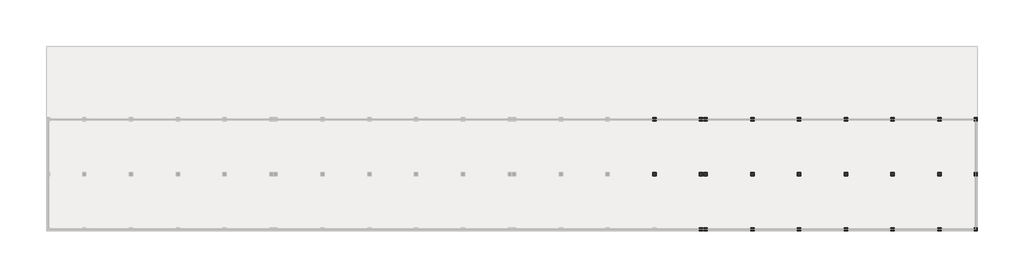
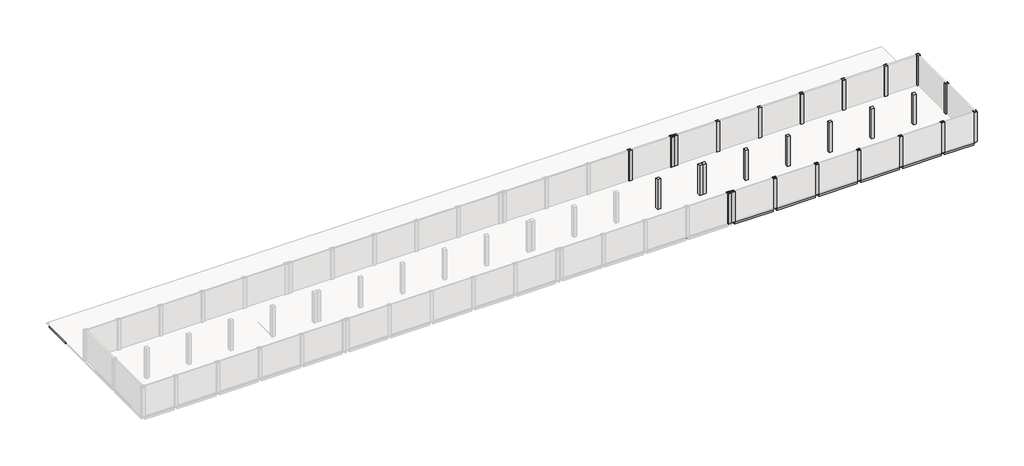
# One storey, part 3 of 4: 52 beams, 26 columns.
"""IFC4 building model written with IfcOpenShell, lengths in millimetres."""

import ifcopenshell
import ifcopenshell.guid

model = None  # the IFC model being written
_history = None  # IfcOwnerHistory: only IFC2X3 demands one
_inside = {}  # id of a spatial element -> (the spatial element, [elements in it])
_under = {}  # id of a project, library or spatial element -> (it, [spatial elements below it])
_declared = {}  # id of a project -> (the project, [libraries it declares])
_typed = {}  # id of a type object -> (the type object, [elements of that type])
_made_of = {}  # id of a material, layer set ... -> (it, [elements and type objects made of it])


def new_model(schema):
    """Start an empty IFC model of exactly this schema.

    Asked for "IFC4X3", IfcOpenShell would pick the latest addendum, in which some entities
    have other attributes; the version numbers below select the first issue.
    IFC2X3 requires an IfcOwnerHistory on every rooted entity: one is made here for all.
    """
    global model, _history
    if schema == "IFC4X3":
        model = ifcopenshell.file(schema_version=(4, 3, 0, 0))
    else:
        model = ifcopenshell.file(schema=schema)
    _inside.clear()
    _under.clear()
    _declared.clear()
    _typed.clear()
    _made_of.clear()
    _history = None
    if model.schema == "IFC2X3":
        org = make("IfcOrganization", Name="unknown")
        user = make(
            "IfcPersonAndOrganization",
            ThePerson=make("IfcPerson", FamilyName="unknown"),
            TheOrganization=org,
        )
        app = make(
            "IfcApplication",
            ApplicationDeveloper=org,
            Version="unknown",
            ApplicationFullName="unknown",
            ApplicationIdentifier="unknown",
        )
        _history = make(
            "IfcOwnerHistory",
            OwningUser=user,
            OwningApplication=app,
            ChangeAction="ADDED",
            CreationDate=0,
        )
    return model


def make(cls, **values):
    """One entity of the class cls with the attributes given. An attribute that is None is left unset."""
    return model.create_entity(
        cls, **{name: value for name, value in values.items() if value is not None}
    )


def rooted(cls, **values):
    """An entity with a GlobalId (a new one), such as an element, a storey or a relation."""
    return make(cls, GlobalId=ifcopenshell.guid.new(), OwnerHistory=_history, **values)


def si_unit(unit_type, name, prefix=None):
    """IfcSIUnit, for example si_unit("LENGTHUNIT", "METRE", prefix="MILLI")."""
    return make("IfcSIUnit", UnitType=unit_type, Prefix=prefix, Name=name)


def assignment(units):
    """IfcUnitAssignment: the units of a project."""
    return None if units is None else make("IfcUnitAssignment", Units=units)


def point(xyz):
    """IfcCartesianPoint."""
    return None if xyz is None else make("IfcCartesianPoint", Coordinates=xyz)


def direction(xyz):
    """IfcDirection."""
    return None if xyz is None else make("IfcDirection", DirectionRatios=xyz)


def frame(location, z_axis=None, x_axis=None):
    """IfcAxis2Placement3D, a coordinate frame: its origin and axes. An axis left out is left unset."""
    return make(
        "IfcAxis2Placement3D",
        Location=point(location),
        Axis=direction(z_axis),
        RefDirection=direction(x_axis),
    )


def origin():
    """The frame at (0, 0, 0) with its axes left unset."""
    return frame((0.0, 0.0, 0.0))


def place(relative_to, where):
    """IfcLocalPlacement: puts the frame where relative to a parent placement (None: the world)."""
    return make(
        "IfcLocalPlacement", PlacementRelTo=relative_to, RelativePlacement=where
    )


def context(
    kind, dimensions, precision=None, world=None, true_north=None, identifier=None
):
    """IfcGeometricRepresentationContext, for example the 3D "Model" context."""
    return make(
        "IfcGeometricRepresentationContext",
        ContextIdentifier=identifier,
        ContextType=kind,
        CoordinateSpaceDimension=dimensions,
        Precision=precision,
        WorldCoordinateSystem=world,
        TrueNorth=true_north,
    )


def project(units=None, contexts=None):
    """IfcProject with its units and contexts."""
    return rooted(
        "IfcProject",
        Name="project",
        RepresentationContexts=contexts,
        UnitsInContext=assignment(units),
    )


def spatial(cls, under=None, at=None, **own):
    """A site, building, storey or space (cls), placed at a placement, below another one or the project."""
    s = rooted(cls, ObjectPlacement=at, **own)
    if under is not None:
        _under.setdefault(under.id(), (under, []))[1].append(s)
    return s


def polyline(points):
    """IfcPolyline through the points."""
    return make("IfcPolyline", Points=[point(p) for p in points])


def outline(outer, holes=None, kind="AREA"):
    """IfcArbitraryClosedProfileDef: a profile drawn as a closed curve; with holes, ...WithVoids."""
    if holes is None:
        return make("IfcArbitraryClosedProfileDef", ProfileType=kind, OuterCurve=outer)
    return make(
        "IfcArbitraryProfileDefWithVoids",
        ProfileType=kind,
        OuterCurve=outer,
        InnerCurves=holes,
    )


def extrude(swept, where, along, depth):
    """IfcExtrudedAreaSolid: the profile swept, set in the frame where, extruded along a direction by depth."""
    return make(
        "IfcExtrudedAreaSolid",
        SweptArea=swept,
        Position=where,
        ExtrudedDirection=direction(along),
        Depth=depth,
    )


def shape(context_of_items, identifier, shape_type, items):
    """IfcShapeRepresentation: the items that make up one representation, for example the "Body"."""
    return make(
        "IfcShapeRepresentation",
        ContextOfItems=context_of_items,
        RepresentationIdentifier=identifier,
        RepresentationType=shape_type,
        Items=items,
    )


def made_of(thing, what):
    """Note that an element or type object is made of a material, layer set ...; save() writes the relation."""
    if what is not None:
        _made_of.setdefault(what.id(), (what, []))[1].append(thing)
    return thing


def element(
    cls,
    number,
    at=None,
    inside=None,
    cuts=None,
    type_object=None,
    material=None,
    context=None,
    identifier="Body",
    shape_type=None,
    held_by="IfcProductDefinitionShape",
    body=None,
    shapes=None,
    **own,
):
    """One element of the class cls, such as IfcWall. Its Tag is "e" and its number.

    at: its placement. inside: the storey or other place that contains it. cuts: it is an
    opening in that element (IfcRelVoidsElement). A single representation is given by context,
    identifier, shape_type and body (its items); several are given by shapes. held_by: the class
    of the entity that holds the representations. save() writes the other relations.
    """
    e = rooted(cls, Tag="e%d" % number, ObjectPlacement=at, **own)
    if body is not None:
        shapes = [shape(context, identifier, shape_type, body)]
    if shapes is not None:
        e.Representation = make(held_by, Representations=shapes)
    if inside is not None:
        _inside.setdefault(inside.id(), (inside, []))[1].append(e)
    if cuts is not None:
        rooted(
            "IfcRelVoidsElement", RelatingBuildingElement=cuts, RelatedOpeningElement=e
        )
    if type_object is not None:
        _typed.setdefault(type_object.id(), (type_object, []))[1].append(e)
    return made_of(e, material)


def aggregate(whole, parts):
    """IfcRelAggregates: a whole, such as a stair, and the parts it consists of."""
    return rooted("IfcRelAggregates", RelatingObject=whole, RelatedObjects=parts)


def save(model, path):
    """Write the relations noted so far, then the file.

    IfcRelAggregates (storeys below a building ...), IfcRelContainedInSpatialStructure (elements
    in a storey), IfcRelDefinesByType, IfcRelAssociatesMaterial and IfcRelDeclares: one each for
    every whole, place, type object, material and project.
    """
    for whole, parts in _under.values():
        aggregate(whole, parts)
    for where, things in _inside.values():
        rooted(
            "IfcRelContainedInSpatialStructure",
            RelatedElements=things,
            RelatingStructure=where,
        )
    for kind, things in _typed.values():
        rooted("IfcRelDefinesByType", RelatedObjects=things, RelatingType=kind)
    for what, things in _made_of.values():
        rooted("IfcRelAssociatesMaterial", RelatedObjects=things, RelatingMaterial=what)
    for by, libraries in _declared.values():
        rooted("IfcRelDeclares", RelatingContext=by, RelatedDefinitions=libraries)
    model.write(path)


model = new_model("IFC4")

# Units and contexts
model_context = context("Model", 3, world=origin())
ifc_project = project(units=[si_unit("LENGTHUNIT", "METRE", prefix="MILLI")], contexts=[model_context])

# Site, building, storey
site = spatial("IfcSite", under=ifc_project)
building = spatial("IfcBuilding", under=site)
storey = spatial("IfcBuildingStorey", under=building, Name="03_T.O.C_1", Elevation=6949.9618634)

# Beams
placement = place(None, origin())
element("IfcBeam", 1, ObjectType="RC Beam_Rectangular : H_SB_AR_S16_B300xH600", at=placement, inside=storey, context=model_context, shape_type="SweptSolid", body=[
    extrude(outline(polyline([(93930.0, -6150.4791411), (93930.0, -5850.4791411), (101530.0, -5850.4791411), (101530.0, -6150.4791411), (93930.0, -6150.4791411)])), frame((0.0, 0.0, 6349.9618634), z_axis=(0.0, 0.0, 1.0), x_axis=(1.0, 0.0, 0.0)), (0.0, 0.0, 1.0), 499.0),
])
element("IfcBeam", 2, ObjectType="RC Beam_Rectangular : H_SB_AR_S16_B300xH600", at=placement, inside=storey, context=model_context, shape_type="SweptSolid", body=[
    extrude(outline(polyline([(102130.0, -6150.4791411), (102130.0, -5850.4791411), (109730.0, -5850.4791411), (109730.0, -6150.4791411), (102130.0, -6150.4791411)])), frame((0.0, 0.0, 6349.9618634), z_axis=(0.0, 0.0, 1.0), x_axis=(1.0, 0.0, 0.0)), (0.0, 0.0, 1.0), 499.0),
])
element("IfcBeam", 3, ObjectType="RC Beam_Rectangular : H_SB_AR_S16_B300xH600", at=placement, inside=storey, context=model_context, shape_type="SweptSolid", body=[
    extrude(outline(polyline([(110330.0, -6150.4791411), (110330.0, -5850.4791411), (110480.0, -5850.4791411), (110480.0, -6150.4791411), (110330.0, -6150.4791411)])), frame((0.0, 0.0, 6349.9618634), z_axis=(0.0, 0.0, 1.0), x_axis=(1.0, 0.0, 0.0)), (0.0, 0.0, 1.0), 499.0),
])
element("IfcBeam", 4, ObjectType="RC Beam_Rectangular : H_SB_AR_S16_B300xH600", at=placement, inside=storey, context=model_context, shape_type="SweptSolid", body=[
    extrude(outline(polyline([(111080.0, -6150.4791411), (111080.0, -5850.4791411), (118680.0, -5850.4791411), (118680.0, -6150.4791411), (111080.0, -6150.4791411)])), frame((0.0, 0.0, 6349.9618634), z_axis=(0.0, 0.0, 1.0), x_axis=(1.0, 0.0, 0.0)), (0.0, 0.0, 1.0), 499.0),
])
element("IfcBeam", 5, ObjectType="RC Beam_Rectangular : H_SB_AR_S16_B300xH600", at=placement, inside=storey, context=model_context, shape_type="SweptSolid", body=[
    extrude(outline(polyline([(119280.0, -6150.4791411), (119280.0, -5850.4791411), (126880.0, -5850.4791411), (126880.0, -6150.4791411), (119280.0, -6150.4791411)])), frame((0.0, 0.0, 6349.9618634), z_axis=(0.0, 0.0, 1.0), x_axis=(1.0, 0.0, 0.0)), (0.0, 0.0, 1.0), 499.0),
])
element("IfcBeam", 6, ObjectType="RC Beam_Rectangular : H_SB_AR_S16_B300xH600", at=placement, inside=storey, context=model_context, shape_type="SweptSolid", body=[
    extrude(outline(polyline([(127480.0, -6150.4791411), (127480.0, -5850.4791411), (135080.0, -5850.4791411), (135080.0, -6150.4791411), (127480.0, -6150.4791411)])), frame((0.0, 0.0, 6349.9618634), z_axis=(0.0, 0.0, 1.0), x_axis=(1.0, 0.0, 0.0)), (0.0, 0.0, 1.0), 499.0),
])
element("IfcBeam", 7, ObjectType="RC Beam_Rectangular : H_SB_AR_S16_B300xH600", at=placement, inside=storey, context=model_context, shape_type="SweptSolid", body=[
    extrude(outline(polyline([(135680.0, -6150.4791411), (135680.0, -5850.4791411), (143280.0, -5850.4791411), (143280.0, -6150.4791411), (135680.0, -6150.4791411)])), frame((0.0, 0.0, 6349.9618634), z_axis=(0.0, 0.0, 1.0), x_axis=(1.0, 0.0, 0.0)), (0.0, 0.0, 1.0), 499.0),
])
element("IfcBeam", 8, ObjectType="RC Beam_Rectangular : H_SB_AR_S16_B300xH600", at=placement, inside=storey, context=model_context, shape_type="SweptSolid", body=[
    extrude(outline(polyline([(143880.0, -6150.4791411), (143880.0, -5850.4791411), (151480.0, -5850.4791411), (151480.0, -6150.4791411), (143880.0, -6150.4791411)])), frame((0.0, 0.0, 6349.9618634), z_axis=(0.0, 0.0, 1.0), x_axis=(1.0, 0.0, 0.0)), (0.0, 0.0, 1.0), 499.0),
])
element("IfcBeam", 9, ObjectType="RC Beam_Rectangular : H_SB_AR_S16_B300xH600", at=placement, inside=storey, context=model_context, shape_type="SweptSolid", body=[
    extrude(outline(polyline([(152080.0, -6150.4791411), (152080.0, -5850.4791411), (157830.0, -5850.4791411), (157830.0, -6150.4791411), (152080.0, -6150.4791411)])), frame((0.0, 0.0, 6349.9618634), z_axis=(0.0, 0.0, 1.0), x_axis=(1.0, 0.0, 0.0)), (0.0, 0.0, 1.0), 499.0),
])
element("IfcBeam", 10, ObjectType="RC Beam_Rectangular : H_SB_AR_S16_B300xH600", at=placement, inside=storey, context=model_context, shape_type="SweptSolid", body=[
    extrude(outline(polyline([(93930.0, -15800.4791411), (93930.0, -15500.4791411), (101530.0, -15500.4791411), (101530.0, -15800.4791411), (93930.0, -15800.4791411)])), frame((0.0, 0.0, 6349.9618634), z_axis=(0.0, 0.0, 1.0), x_axis=(1.0, 0.0, 0.0)), (0.0, 0.0, 1.0), 499.0),
])
element("IfcBeam", 11, ObjectType="RC Beam_Rectangular : H_SB_AR_S16_B300xH600", at=placement, inside=storey, context=model_context, shape_type="SweptSolid", body=[
    extrude(outline(polyline([(102130.0, -15800.4791411), (102130.0, -15500.4791411), (109730.0, -15500.4791411), (109730.0, -15800.4791411), (102130.0, -15800.4791411)])), frame((0.0, 0.0, 6349.9618634), z_axis=(0.0, 0.0, 1.0), x_axis=(1.0, 0.0, 0.0)), (0.0, 0.0, 1.0), 499.0),
])
element("IfcBeam", 12, ObjectType="RC Beam_Rectangular : H_SB_AR_S16_B300xH600", at=placement, inside=storey, context=model_context, shape_type="SweptSolid", body=[
    extrude(outline(polyline([(110330.0, -15800.4791411), (110330.0, -15500.4791411), (110480.0, -15500.4791411), (110480.0, -15800.4791411), (110330.0, -15800.4791411)])), frame((0.0, 0.0, 6349.9618634), z_axis=(0.0, 0.0, 1.0), x_axis=(1.0, 0.0, 0.0)), (0.0, 0.0, 1.0), 499.0),
])
element("IfcBeam", 13, ObjectType="RC Beam_Rectangular : H_SB_AR_S16_B300xH600", at=placement, inside=storey, context=model_context, shape_type="SweptSolid", body=[
    extrude(outline(polyline([(111080.0, -15800.4791411), (111080.0, -15500.4791411), (118680.0, -15500.4791411), (118680.0, -15800.4791411), (111080.0, -15800.4791411)])), frame((0.0, 0.0, 6349.9618634), z_axis=(0.0, 0.0, 1.0), x_axis=(1.0, 0.0, 0.0)), (0.0, 0.0, 1.0), 499.0),
])
element("IfcBeam", 14, ObjectType="RC Beam_Rectangular : H_SB_AR_S16_B300xH600", at=placement, inside=storey, context=model_context, shape_type="SweptSolid", body=[
    extrude(outline(polyline([(119280.0, -15800.4791411), (119280.0, -15500.4791411), (126880.0, -15500.4791411), (126880.0, -15800.4791411), (119280.0, -15800.4791411)])), frame((0.0, 0.0, 6349.9618634), z_axis=(0.0, 0.0, 1.0), x_axis=(1.0, 0.0, 0.0)), (0.0, 0.0, 1.0), 499.0),
])
element("IfcBeam", 15, ObjectType="RC Beam_Rectangular : H_SB_AR_S16_B300xH600", at=placement, inside=storey, context=model_context, shape_type="SweptSolid", body=[
    extrude(outline(polyline([(127480.0, -15800.4791411), (127480.0, -15500.4791411), (135080.0, -15500.4791411), (135080.0, -15800.4791411), (127480.0, -15800.4791411)])), frame((0.0, 0.0, 6349.9618634), z_axis=(0.0, 0.0, 1.0), x_axis=(1.0, 0.0, 0.0)), (0.0, 0.0, 1.0), 499.0),
])
element("IfcBeam", 16, ObjectType="RC Beam_Rectangular : H_SB_AR_S16_B300xH600", at=placement, inside=storey, context=model_context, shape_type="SweptSolid", body=[
    extrude(outline(polyline([(135680.0, -15800.4791411), (135680.0, -15500.4791411), (143280.0, -15500.4791411), (143280.0, -15800.4791411), (135680.0, -15800.4791411)])), frame((0.0, 0.0, 6349.9618634), z_axis=(0.0, 0.0, 1.0), x_axis=(1.0, 0.0, 0.0)), (0.0, 0.0, 1.0), 499.0),
])
element("IfcBeam", 17, ObjectType="RC Beam_Rectangular : H_SB_AR_S16_B300xH600", at=placement, inside=storey, context=model_context, shape_type="SweptSolid", body=[
    extrude(outline(polyline([(143880.0, -15800.4791411), (143880.0, -15500.4791411), (151480.0, -15500.4791411), (151480.0, -15800.4791411), (143880.0, -15800.4791411)])), frame((0.0, 0.0, 6349.9618634), z_axis=(0.0, 0.0, 1.0), x_axis=(1.0, 0.0, 0.0)), (0.0, 0.0, 1.0), 499.0),
])
element("IfcBeam", 18, ObjectType="RC Beam_Rectangular : H_SB_AR_S16_B300xH600", at=placement, inside=storey, context=model_context, shape_type="SweptSolid", body=[
    extrude(outline(polyline([(152080.0, -15800.4791411), (152080.0, -15500.4791411), (157830.0, -15500.4791411), (157830.0, -15800.4791411), (152080.0, -15800.4791411)])), frame((0.0, 0.0, 6349.9618634), z_axis=(0.0, 0.0, 1.0), x_axis=(1.0, 0.0, 0.0)), (0.0, 0.0, 1.0), 499.0),
])
element("IfcBeam", 19, ObjectType="RC Beam_Rectangular : H_SB_AR_S16_B300xH600", at=placement, inside=storey, context=model_context, shape_type="SweptSolid", body=[
    extrude(outline(polyline([(111080.0, -25450.4791411), (111080.0, -25150.4791411), (118680.0, -25150.4791411), (118680.0, -25450.4791411), (111080.0, -25450.4791411)])), frame((0.0, 0.0, 6349.9618634), z_axis=(0.0, 0.0, 1.0), x_axis=(1.0, 0.0, 0.0)), (0.0, 0.0, 1.0), 499.0),
])
element("IfcBeam", 20, ObjectType="RC Beam_Rectangular : H_SB_AR_S16_B300xH600", at=placement, inside=storey, context=model_context, shape_type="SweptSolid", body=[
    extrude(outline(polyline([(119280.0, -25450.4791411), (119280.0, -25150.4791411), (126880.0, -25150.4791411), (126880.0, -25450.4791411), (119280.0, -25450.4791411)])), frame((0.0, 0.0, 6349.9618634), z_axis=(0.0, 0.0, 1.0), x_axis=(1.0, 0.0, 0.0)), (0.0, 0.0, 1.0), 499.0),
])
element("IfcBeam", 21, ObjectType="RC Beam_Rectangular : H_SB_AR_S16_B300xH600", at=placement, inside=storey, context=model_context, shape_type="SweptSolid", body=[
    extrude(outline(polyline([(127480.0, -25450.4791411), (127480.0, -25150.4791411), (135080.0, -25150.4791411), (135080.0, -25450.4791411), (127480.0, -25450.4791411)])), frame((0.0, 0.0, 6349.9618634), z_axis=(0.0, 0.0, 1.0), x_axis=(1.0, 0.0, 0.0)), (0.0, 0.0, 1.0), 499.0),
])
element("IfcBeam", 22, ObjectType="RC Beam_Rectangular : H_SB_AR_S16_B300xH600", at=placement, inside=storey, context=model_context, shape_type="SweptSolid", body=[
    extrude(outline(polyline([(135680.0, -25450.4791411), (135680.0, -25150.4791411), (143280.0, -25150.4791411), (143280.0, -25450.4791411), (135680.0, -25450.4791411)])), frame((0.0, 0.0, 6349.9618634), z_axis=(0.0, 0.0, 1.0), x_axis=(1.0, 0.0, 0.0)), (0.0, 0.0, 1.0), 499.0),
])
element("IfcBeam", 23, ObjectType="RC Beam_Rectangular : H_SB_AR_S16_B300xH600", at=placement, inside=storey, context=model_context, shape_type="SweptSolid", body=[
    extrude(outline(polyline([(143880.0, -25450.4791411), (143880.0, -25150.4791411), (151480.0, -25150.4791411), (151480.0, -25450.4791411), (143880.0, -25450.4791411)])), frame((0.0, 0.0, 6349.9618634), z_axis=(0.0, 0.0, 1.0), x_axis=(1.0, 0.0, 0.0)), (0.0, 0.0, 1.0), 499.0),
])
element("IfcBeam", 24, ObjectType="RC Beam_Rectangular : H_SB_AR_S16_B300xH600", at=placement, inside=storey, context=model_context, shape_type="SweptSolid", body=[
    extrude(outline(polyline([(152080.0, -25450.4791411), (152080.0, -25150.4791411), (157830.0, -25150.4791411), (157830.0, -25450.4791411), (152080.0, -25450.4791411)])), frame((0.0, 0.0, 6349.9618634), z_axis=(0.0, 0.0, 1.0), x_axis=(1.0, 0.0, 0.0)), (0.0, 0.0, 1.0), 499.0),
])
element("IfcBeam", 25, ObjectType="RC Beam_Rectangular : H_SB_AR_S16_B300xH600", at=placement, inside=storey, context=model_context, shape_type="SweptSolid", body=[
    extrude(outline(polyline([(-4220.0, 549.5208589), (-4520.0, 549.5208589), (-4520.0, 6199.5208589), (-4220.0, 6199.5208589), (-4220.0, 549.5208589)])), frame((0.0, 0.0, 6349.9618634), z_axis=(0.0, 0.0, 1.0), x_axis=(1.0, 0.0, 0.0)), (0.0, 0.0, 1.0), 499.0),
])
element("IfcBeam", 26, ObjectType="RC Beam_Rectangular : H_SB_AR_S16_B300xH600", at=placement, inside=storey, context=model_context, shape_type="SweptSolid", body=[
    extrude(outline(polyline([(101680.0, -15950.4791411), (101980.0, -15950.4791411), (101980.0, -25000.4791411), (101680.0, -25000.4791411), (101680.0, -15950.4791411)])), frame((0.0, 0.0, 6349.9618634), z_axis=(0.0, 0.0, 1.0), x_axis=(1.0, 0.0, 0.0)), (0.0, 0.0, 1.0), 499.0),
])
element("IfcBeam", 27, ObjectType="RC Beam_Rectangular : H_SB_AR_S16_B300xH600", at=placement, inside=storey, context=model_context, shape_type="SweptSolid", body=[
    extrude(outline(polyline([(101680.0, -6300.4791411), (101980.0, -6300.4791411), (101980.0, -15350.4791411), (101680.0, -15350.4791411), (101680.0, -6300.4791411)])), frame((0.0, 0.0, 6349.9618634), z_axis=(0.0, 0.0, 1.0), x_axis=(1.0, 0.0, 0.0)), (0.0, 0.0, 1.0), 499.0),
])
element("IfcBeam", 28, ObjectType="RC Beam_Rectangular : H_SB_AR_S16_B300xH600", at=placement, inside=storey, context=model_context, shape_type="SweptSolid", body=[
    extrude(outline(polyline([(101680.0, 99.5208589), (101980.0, 99.5208589), (101980.0, -5700.4791411), (101680.0, -5700.4791411), (101680.0, 99.5208589)])), frame((0.0, 0.0, 6349.9618634), z_axis=(0.0, 0.0, 1.0), x_axis=(1.0, 0.0, 0.0)), (0.0, 0.0, 1.0), 499.0),
])
element("IfcBeam", 29, ObjectType="RC Beam_Rectangular : H_SB_AR_S16_B300xH600", at=placement, inside=storey, context=model_context, shape_type="SweptSolid", body=[
    extrude(outline(polyline([(109880.0, -15950.4791411), (110180.0, -15950.4791411), (110180.0, -25000.4791411), (109880.0, -25000.4791411), (109880.0, -15950.4791411)])), frame((0.0, 0.0, 6349.9618634), z_axis=(0.0, 0.0, 1.0), x_axis=(1.0, 0.0, 0.0)), (0.0, 0.0, 1.0), 499.0),
])
element("IfcBeam", 30, ObjectType="RC Beam_Rectangular : H_SB_AR_S16_B300xH600", at=placement, inside=storey, context=model_context, shape_type="SweptSolid", body=[
    extrude(outline(polyline([(109880.0, -6300.4791411), (110180.0, -6300.4791411), (110180.0, -15350.4791411), (109880.0, -15350.4791411), (109880.0, -6300.4791411)])), frame((0.0, 0.0, 6349.9618634), z_axis=(0.0, 0.0, 1.0), x_axis=(1.0, 0.0, 0.0)), (0.0, 0.0, 1.0), 499.0),
])
element("IfcBeam", 31, ObjectType="RC Beam_Rectangular : H_SB_AR_S16_B300xH600", at=placement, inside=storey, context=model_context, shape_type="SweptSolid", body=[
    extrude(outline(polyline([(109880.0, -50.4791411), (110180.0, -50.4791411), (110180.0, -5700.4791411), (109880.0, -5700.4791411), (109880.0, -50.4791411)])), frame((0.0, 0.0, 6349.9618634), z_axis=(0.0, 0.0, 1.0), x_axis=(1.0, 0.0, 0.0)), (0.0, 0.0, 1.0), 499.0),
])
element("IfcBeam", 32, ObjectType="RC Beam_Rectangular : H_SB_AR_S16_B300xH600", at=placement, inside=storey, context=model_context, shape_type="SweptSolid", body=[
    extrude(outline(polyline([(110630.0, -15950.4791411), (110930.0, -15950.4791411), (110930.0, -25000.4791411), (110630.0, -25000.4791411), (110630.0, -15950.4791411)])), frame((0.0, 0.0, 6349.9618634), z_axis=(0.0, 0.0, 1.0), x_axis=(1.0, 0.0, 0.0)), (0.0, 0.0, 1.0), 499.0),
])
element("IfcBeam", 33, ObjectType="RC Beam_Rectangular : H_SB_AR_S16_B300xH600", at=placement, inside=storey, context=model_context, shape_type="SweptSolid", body=[
    extrude(outline(polyline([(110630.0, -6300.4791411), (110930.0, -6300.4791411), (110930.0, -15350.4791411), (110630.0, -15350.4791411), (110630.0, -6300.4791411)])), frame((0.0, 0.0, 6349.9618634), z_axis=(0.0, 0.0, 1.0), x_axis=(1.0, 0.0, 0.0)), (0.0, 0.0, 1.0), 499.0),
])
element("IfcBeam", 34, ObjectType="RC Beam_Rectangular : H_SB_AR_S16_B300xH600", at=placement, inside=storey, context=model_context, shape_type="SweptSolid", body=[
    extrude(outline(polyline([(110630.0, -50.4791411), (110930.0, -50.4791411), (110930.0, -5700.4791411), (110630.0, -5700.4791411), (110630.0, -50.4791411)])), frame((0.0, 0.0, 6349.9618634), z_axis=(0.0, 0.0, 1.0), x_axis=(1.0, 0.0, 0.0)), (0.0, 0.0, 1.0), 499.0),
])
element("IfcBeam", 35, ObjectType="RC Beam_Rectangular : H_SB_AR_S16_B300xH600", at=placement, inside=storey, context=model_context, shape_type="SweptSolid", body=[
    extrude(outline(polyline([(118830.0, -15950.4791411), (119130.0, -15950.4791411), (119130.0, -25000.4791411), (118830.0, -25000.4791411), (118830.0, -15950.4791411)])), frame((0.0, 0.0, 6349.9618634), z_axis=(0.0, 0.0, 1.0), x_axis=(1.0, 0.0, 0.0)), (0.0, 0.0, 1.0), 499.0),
])
element("IfcBeam", 36, ObjectType="RC Beam_Rectangular : H_SB_AR_S16_B300xH600", at=placement, inside=storey, context=model_context, shape_type="SweptSolid", body=[
    extrude(outline(polyline([(118830.0, -6300.4791411), (119130.0, -6300.4791411), (119130.0, -15350.4791411), (118830.0, -15350.4791411), (118830.0, -6300.4791411)])), frame((0.0, 0.0, 6349.9618634), z_axis=(0.0, 0.0, 1.0), x_axis=(1.0, 0.0, 0.0)), (0.0, 0.0, 1.0), 499.0),
])
element("IfcBeam", 37, ObjectType="RC Beam_Rectangular : H_SB_AR_S16_B300xH600", at=placement, inside=storey, context=model_context, shape_type="SweptSolid", body=[
    extrude(outline(polyline([(118830.0, -50.4791411), (119130.0, -50.4791411), (119130.0, -5700.4791411), (118830.0, -5700.4791411), (118830.0, -50.4791411)])), frame((0.0, 0.0, 6349.9618634), z_axis=(0.0, 0.0, 1.0), x_axis=(1.0, 0.0, 0.0)), (0.0, 0.0, 1.0), 499.0),
])
element("IfcBeam", 38, ObjectType="RC Beam_Rectangular : H_SB_AR_S16_B300xH600", at=placement, inside=storey, context=model_context, shape_type="SweptSolid", body=[
    extrude(outline(polyline([(127030.0, -15950.4791411), (127330.0, -15950.4791411), (127330.0, -25000.4791411), (127030.0, -25000.4791411), (127030.0, -15950.4791411)])), frame((0.0, 0.0, 6349.9618634), z_axis=(0.0, 0.0, 1.0), x_axis=(1.0, 0.0, 0.0)), (0.0, 0.0, 1.0), 499.0),
])
element("IfcBeam", 39, ObjectType="RC Beam_Rectangular : H_SB_AR_S16_B300xH600", at=placement, inside=storey, context=model_context, shape_type="SweptSolid", body=[
    extrude(outline(polyline([(127030.0, -6300.4791411), (127330.0, -6300.4791411), (127330.0, -15350.4791411), (127030.0, -15350.4791411), (127030.0, -6300.4791411)])), frame((0.0, 0.0, 6349.9618634), z_axis=(0.0, 0.0, 1.0), x_axis=(1.0, 0.0, 0.0)), (0.0, 0.0, 1.0), 499.0),
])
element("IfcBeam", 40, ObjectType="RC Beam_Rectangular : H_SB_AR_S16_B300xH600", at=placement, inside=storey, context=model_context, shape_type="SweptSolid", body=[
    extrude(outline(polyline([(127030.0, -50.4791411), (127330.0, -50.4791411), (127330.0, -5700.4791411), (127030.0, -5700.4791411), (127030.0, -50.4791411)])), frame((0.0, 0.0, 6349.9618634), z_axis=(0.0, 0.0, 1.0), x_axis=(1.0, 0.0, 0.0)), (0.0, 0.0, 1.0), 499.0),
])
element("IfcBeam", 41, ObjectType="RC Beam_Rectangular : H_SB_AR_S16_B300xH600", at=placement, inside=storey, context=model_context, shape_type="SweptSolid", body=[
    extrude(outline(polyline([(135230.0, -15950.4791411), (135530.0, -15950.4791411), (135530.0, -25000.4791411), (135230.0, -25000.4791411), (135230.0, -15950.4791411)])), frame((0.0, 0.0, 6349.9618634), z_axis=(0.0, 0.0, 1.0), x_axis=(1.0, 0.0, 0.0)), (0.0, 0.0, 1.0), 499.0),
])
element("IfcBeam", 42, ObjectType="RC Beam_Rectangular : H_SB_AR_S16_B300xH600", at=placement, inside=storey, context=model_context, shape_type="SweptSolid", body=[
    extrude(outline(polyline([(135230.0, -6300.4791411), (135530.0, -6300.4791411), (135530.0, -15350.4791411), (135230.0, -15350.4791411), (135230.0, -6300.4791411)])), frame((0.0, 0.0, 6349.9618634), z_axis=(0.0, 0.0, 1.0), x_axis=(1.0, 0.0, 0.0)), (0.0, 0.0, 1.0), 499.0),
])
element("IfcBeam", 43, ObjectType="RC Beam_Rectangular : H_SB_AR_S16_B300xH600", at=placement, inside=storey, context=model_context, shape_type="SweptSolid", body=[
    extrude(outline(polyline([(135230.0, -50.4791411), (135530.0, -50.4791411), (135530.0, -5700.4791411), (135230.0, -5700.4791411), (135230.0, -50.4791411)])), frame((0.0, 0.0, 6349.9618634), z_axis=(0.0, 0.0, 1.0), x_axis=(1.0, 0.0, 0.0)), (0.0, 0.0, 1.0), 499.0),
])
element("IfcBeam", 44, ObjectType="RC Beam_Rectangular : H_SB_AR_S16_B300xH600", at=placement, inside=storey, context=model_context, shape_type="SweptSolid", body=[
    extrude(outline(polyline([(143430.0, -15950.4791411), (143730.0, -15950.4791411), (143730.0, -25000.4791411), (143430.0, -25000.4791411), (143430.0, -15950.4791411)])), frame((0.0, 0.0, 6349.9618634), z_axis=(0.0, 0.0, 1.0), x_axis=(1.0, 0.0, 0.0)), (0.0, 0.0, 1.0), 499.0),
])
element("IfcBeam", 45, ObjectType="RC Beam_Rectangular : H_SB_AR_S16_B300xH600", at=placement, inside=storey, context=model_context, shape_type="SweptSolid", body=[
    extrude(outline(polyline([(143430.0, -6300.4791411), (143730.0, -6300.4791411), (143730.0, -15350.4791411), (143430.0, -15350.4791411), (143430.0, -6300.4791411)])), frame((0.0, 0.0, 6349.9618634), z_axis=(0.0, 0.0, 1.0), x_axis=(1.0, 0.0, 0.0)), (0.0, 0.0, 1.0), 499.0),
])
element("IfcBeam", 46, ObjectType="RC Beam_Rectangular : H_SB_AR_S16_B300xH600", at=placement, inside=storey, context=model_context, shape_type="SweptSolid", body=[
    extrude(outline(polyline([(143430.0, -50.4791411), (143730.0, -50.4791411), (143730.0, -5700.4791411), (143430.0, -5700.4791411), (143430.0, -50.4791411)])), frame((0.0, 0.0, 6349.9618634), z_axis=(0.0, 0.0, 1.0), x_axis=(1.0, 0.0, 0.0)), (0.0, 0.0, 1.0), 499.0),
])
element("IfcBeam", 47, ObjectType="RC Beam_Rectangular : H_SB_AR_S16_B300xH600", at=placement, inside=storey, context=model_context, shape_type="SweptSolid", body=[
    extrude(outline(polyline([(151630.0, -15950.4791411), (151930.0, -15950.4791411), (151930.0, -25000.4791411), (151630.0, -25000.4791411), (151630.0, -15950.4791411)])), frame((0.0, 0.0, 6349.9618634), z_axis=(0.0, 0.0, 1.0), x_axis=(1.0, 0.0, 0.0)), (0.0, 0.0, 1.0), 499.0),
])
element("IfcBeam", 48, ObjectType="RC Beam_Rectangular : H_SB_AR_S16_B300xH600", at=placement, inside=storey, context=model_context, shape_type="SweptSolid", body=[
    extrude(outline(polyline([(151630.0, -6300.4791411), (151930.0, -6300.4791411), (151930.0, -15350.4791411), (151630.0, -15350.4791411), (151630.0, -6300.4791411)])), frame((0.0, 0.0, 6349.9618634), z_axis=(0.0, 0.0, 1.0), x_axis=(1.0, 0.0, 0.0)), (0.0, 0.0, 1.0), 499.0),
])
element("IfcBeam", 49, ObjectType="RC Beam_Rectangular : H_SB_AR_S16_B300xH600", at=placement, inside=storey, context=model_context, shape_type="SweptSolid", body=[
    extrude(outline(polyline([(151630.0, -50.4791411), (151930.0, -50.4791411), (151930.0, -5700.4791411), (151630.0, -5700.4791411), (151630.0, -50.4791411)])), frame((0.0, 0.0, 6349.9618634), z_axis=(0.0, 0.0, 1.0), x_axis=(1.0, 0.0, 0.0)), (0.0, 0.0, 1.0), 499.0),
])
element("IfcBeam", 50, ObjectType="RC Beam_Rectangular : H_SB_AR_S16_B300xH600", at=placement, inside=storey, context=model_context, shape_type="SweptSolid", body=[
    extrude(outline(polyline([(157980.0, -15950.4791411), (158280.0, -15950.4791411), (158280.0, -25000.4791411), (157980.0, -25000.4791411), (157980.0, -15950.4791411)])), frame((0.0, 0.0, 6349.9618634), z_axis=(0.0, 0.0, 1.0), x_axis=(1.0, 0.0, 0.0)), (0.0, 0.0, 1.0), 499.0),
])
element("IfcBeam", 51, ObjectType="RC Beam_Rectangular : H_SB_AR_S16_B300xH600", at=placement, inside=storey, context=model_context, shape_type="SweptSolid", body=[
    extrude(outline(polyline([(157980.0, -6300.4791411), (158280.0, -6300.4791411), (158280.0, -15350.4791411), (157980.0, -15350.4791411), (157980.0, -6300.4791411)])), frame((0.0, 0.0, 6349.9618634), z_axis=(0.0, 0.0, 1.0), x_axis=(1.0, 0.0, 0.0)), (0.0, 0.0, 1.0), 499.0),
])
element("IfcBeam", 52, ObjectType="RC Beam_Rectangular : H_SB_AR_S16_B300xH600", at=placement, inside=storey, context=model_context, shape_type="SweptSolid", body=[
    extrude(outline(polyline([(157980.0, -50.4791411), (158280.0, -50.4791411), (158280.0, -5700.4791411), (157980.0, -5700.4791411), (157980.0, -50.4791411)])), frame((0.0, 0.0, 6349.9618634), z_axis=(0.0, 0.0, 1.0), x_axis=(1.0, 0.0, 0.0)), (0.0, 0.0, 1.0), 499.0),
])

# Columns
element("IfcColumn", 53, ObjectType="RC_Column_Rectangular : H_SC_AR_S15_W600xL600", at=placement, inside=storey, context=model_context, shape_type="SweptSolid", body=[
    extrude(outline(polyline([(102130.0, -5700.4791411), (102130.0, -6300.4791411), (101530.0, -6300.4791411), (101530.0, -5700.4791411), (102130.0, -5700.4791411)])), frame((0.0, 0.0, 6949.9618634), z_axis=(0.0, 0.0, 1.0), x_axis=(1.0, 0.0, 0.0)), (0.0, 0.0, 1.0), 6200.0),
])
element("IfcColumn", 54, ObjectType="RC_Column_Rectangular : H_SC_AR_S15_W600xL600", at=placement, inside=storey, context=model_context, shape_type="SweptSolid", body=[
    extrude(outline(polyline([(110330.0, -5700.4791411), (110330.0, -6300.4791411), (109730.0, -6300.4791411), (109730.0, -5700.4791411), (110330.0, -5700.4791411)])), frame((0.0, 0.0, 6949.9618634), z_axis=(0.0, 0.0, 1.0), x_axis=(1.0, 0.0, 0.0)), (0.0, 0.0, 1.0), 6200.0),
])
element("IfcColumn", 55, ObjectType="RC_Column_Rectangular : H_SC_AR_S15_W600xL600", at=placement, inside=storey, context=model_context, shape_type="SweptSolid", body=[
    extrude(outline(polyline([(111080.0, -5700.4791411), (111080.0, -6300.4791411), (110480.0, -6300.4791411), (110480.0, -5700.4791411), (111080.0, -5700.4791411)])), frame((0.0, 0.0, 6949.9618634), z_axis=(0.0, 0.0, 1.0), x_axis=(1.0, 0.0, 0.0)), (0.0, 0.0, 1.0), 6200.0),
])
element("IfcColumn", 56, ObjectType="RC_Column_Rectangular : H_SC_AR_S15_W600xL600", at=placement, inside=storey, context=model_context, shape_type="SweptSolid", body=[
    extrude(outline(polyline([(119280.0, -5700.4791411), (119280.0, -6300.4791411), (118680.0, -6300.4791411), (118680.0, -5700.4791411), (119280.0, -5700.4791411)])), frame((0.0, 0.0, 6949.9618634), z_axis=(0.0, 0.0, 1.0), x_axis=(1.0, 0.0, 0.0)), (0.0, 0.0, 1.0), 6200.0),
])
element("IfcColumn", 57, ObjectType="RC_Column_Rectangular : H_SC_AR_S15_W600xL600", at=placement, inside=storey, context=model_context, shape_type="SweptSolid", body=[
    extrude(outline(polyline([(127480.0, -5700.4791411), (127480.0, -6300.4791411), (126880.0, -6300.4791411), (126880.0, -5700.4791411), (127480.0, -5700.4791411)])), frame((0.0, 0.0, 6949.9618634), z_axis=(0.0, 0.0, 1.0), x_axis=(1.0, 0.0, 0.0)), (0.0, 0.0, 1.0), 6200.0),
])
element("IfcColumn", 58, ObjectType="RC_Column_Rectangular : H_SC_AR_S15_W600xL600", at=placement, inside=storey, context=model_context, shape_type="SweptSolid", body=[
    extrude(outline(polyline([(135680.0, -5700.4791411), (135680.0, -6300.4791411), (135080.0, -6300.4791411), (135080.0, -5700.4791411), (135680.0, -5700.4791411)])), frame((0.0, 0.0, 6949.9618634), z_axis=(0.0, 0.0, 1.0), x_axis=(1.0, 0.0, 0.0)), (0.0, 0.0, 1.0), 6200.0),
])
element("IfcColumn", 59, ObjectType="RC_Column_Rectangular : H_SC_AR_S15_W600xL600", at=placement, inside=storey, context=model_context, shape_type="SweptSolid", body=[
    extrude(outline(polyline([(143880.0, -5700.4791411), (143880.0, -6300.4791411), (143280.0, -6300.4791411), (143280.0, -5700.4791411), (143880.0, -5700.4791411)])), frame((0.0, 0.0, 6949.9618634), z_axis=(0.0, 0.0, 1.0), x_axis=(1.0, 0.0, 0.0)), (0.0, 0.0, 1.0), 6200.0),
])
element("IfcColumn", 60, ObjectType="RC_Column_Rectangular : H_SC_AR_S15_W600xL600", at=placement, inside=storey, context=model_context, shape_type="SweptSolid", body=[
    extrude(outline(polyline([(152080.0, -5700.4791411), (152080.0, -6300.4791411), (151480.0, -6300.4791411), (151480.0, -5700.4791411), (152080.0, -5700.4791411)])), frame((0.0, 0.0, 6949.9618634), z_axis=(0.0, 0.0, 1.0), x_axis=(1.0, 0.0, 0.0)), (0.0, 0.0, 1.0), 6200.0),
])
element("IfcColumn", 61, ObjectType="RC_Column_Rectangular : H_SC_AR_S15_W600xL600", at=placement, inside=storey, context=model_context, shape_type="SweptSolid", body=[
    extrude(outline(polyline([(158430.0, -5700.4791411), (158430.0, -6300.4791411), (157830.0, -6300.4791411), (157830.0, -5700.4791411), (158430.0, -5700.4791411)])), frame((0.0, 0.0, 6949.9618634), z_axis=(0.0, 0.0, 1.0), x_axis=(1.0, 0.0, 0.0)), (0.0, 0.0, 1.0), 6200.0),
])
element("IfcColumn", 62, ObjectType="RC_Column_Rectangular : H_SC_AR_S15_W600xL600", at=placement, inside=storey, context=model_context, shape_type="SweptSolid", body=[
    extrude(outline(polyline([(102130.0, -15350.4791411), (102130.0, -15950.4791411), (101530.0, -15950.4791411), (101530.0, -15350.4791411), (102130.0, -15350.4791411)])), frame((0.0, 0.0, 6949.9618634), z_axis=(0.0, 0.0, 1.0), x_axis=(1.0, 0.0, 0.0)), (0.0, 0.0, 1.0), 6200.0),
])
element("IfcColumn", 63, ObjectType="RC_Column_Rectangular : H_SC_AR_S15_W600xL600", at=placement, inside=storey, context=model_context, shape_type="SweptSolid", body=[
    extrude(outline(polyline([(110330.0, -15350.4791411), (110330.0, -15950.4791411), (109730.0, -15950.4791411), (109730.0, -15350.4791411), (110330.0, -15350.4791411)])), frame((0.0, 0.0, 6949.9618634), z_axis=(0.0, 0.0, 1.0), x_axis=(1.0, 0.0, 0.0)), (0.0, 0.0, 1.0), 6200.0),
])
element("IfcColumn", 64, ObjectType="RC_Column_Rectangular : H_SC_AR_S15_W600xL600", at=placement, inside=storey, context=model_context, shape_type="SweptSolid", body=[
    extrude(outline(polyline([(111080.0, -15350.4791411), (111080.0, -15950.4791411), (110480.0, -15950.4791411), (110480.0, -15350.4791411), (111080.0, -15350.4791411)])), frame((0.0, 0.0, 6949.9618634), z_axis=(0.0, 0.0, 1.0), x_axis=(1.0, 0.0, 0.0)), (0.0, 0.0, 1.0), 6200.0),
])
element("IfcColumn", 65, ObjectType="RC_Column_Rectangular : H_SC_AR_S15_W600xL600", at=placement, inside=storey, context=model_context, shape_type="SweptSolid", body=[
    extrude(outline(polyline([(119280.0, -15350.4791411), (119280.0, -15950.4791411), (118680.0, -15950.4791411), (118680.0, -15350.4791411), (119280.0, -15350.4791411)])), frame((0.0, 0.0, 6949.9618634), z_axis=(0.0, 0.0, 1.0), x_axis=(1.0, 0.0, 0.0)), (0.0, 0.0, 1.0), 6200.0),
])
element("IfcColumn", 66, ObjectType="RC_Column_Rectangular : H_SC_AR_S15_W600xL600", at=placement, inside=storey, context=model_context, shape_type="SweptSolid", body=[
    extrude(outline(polyline([(127480.0, -15350.4791411), (127480.0, -15950.4791411), (126880.0, -15950.4791411), (126880.0, -15350.4791411), (127480.0, -15350.4791411)])), frame((0.0, 0.0, 6949.9618634), z_axis=(0.0, 0.0, 1.0), x_axis=(1.0, 0.0, 0.0)), (0.0, 0.0, 1.0), 6200.0),
])
element("IfcColumn", 67, ObjectType="RC_Column_Rectangular : H_SC_AR_S15_W600xL600", at=placement, inside=storey, context=model_context, shape_type="SweptSolid", body=[
    extrude(outline(polyline([(135680.0, -15350.4791411), (135680.0, -15950.4791411), (135080.0, -15950.4791411), (135080.0, -15350.4791411), (135680.0, -15350.4791411)])), frame((0.0, 0.0, 6949.9618634), z_axis=(0.0, 0.0, 1.0), x_axis=(1.0, 0.0, 0.0)), (0.0, 0.0, 1.0), 6200.0),
])
element("IfcColumn", 68, ObjectType="RC_Column_Rectangular : H_SC_AR_S15_W600xL600", at=placement, inside=storey, context=model_context, shape_type="SweptSolid", body=[
    extrude(outline(polyline([(143880.0, -15350.4791411), (143880.0, -15950.4791411), (143280.0, -15950.4791411), (143280.0, -15350.4791411), (143880.0, -15350.4791411)])), frame((0.0, 0.0, 6949.9618634), z_axis=(0.0, 0.0, 1.0), x_axis=(1.0, 0.0, 0.0)), (0.0, 0.0, 1.0), 6200.0),
])
element("IfcColumn", 69, ObjectType="RC_Column_Rectangular : H_SC_AR_S15_W600xL600", at=placement, inside=storey, context=model_context, shape_type="SweptSolid", body=[
    extrude(outline(polyline([(152080.0, -15350.4791411), (152080.0, -15950.4791411), (151480.0, -15950.4791411), (151480.0, -15350.4791411), (152080.0, -15350.4791411)])), frame((0.0, 0.0, 6949.9618634), z_axis=(0.0, 0.0, 1.0), x_axis=(1.0, 0.0, 0.0)), (0.0, 0.0, 1.0), 6200.0),
])
element("IfcColumn", 70, ObjectType="RC_Column_Rectangular : H_SC_AR_S15_W600xL600", at=placement, inside=storey, context=model_context, shape_type="SweptSolid", body=[
    extrude(outline(polyline([(158430.0, -15350.4791411), (158430.0, -15950.4791411), (157830.0, -15950.4791411), (157830.0, -15350.4791411), (158430.0, -15350.4791411)])), frame((0.0, 0.0, 6949.9618634), z_axis=(0.0, 0.0, 1.0), x_axis=(1.0, 0.0, 0.0)), (0.0, 0.0, 1.0), 6200.0),
])
element("IfcColumn", 71, ObjectType="RC_Column_Rectangular : H_SC_AR_S15_W600xL600", at=placement, inside=storey, context=model_context, shape_type="SweptSolid", body=[
    extrude(outline(polyline([(110330.0, -25000.4791411), (110330.0, -25600.4791411), (109730.0, -25600.4791411), (109730.0, -25000.4791411), (110330.0, -25000.4791411)])), frame((0.0, 0.0, 6949.9618634), z_axis=(0.0, 0.0, 1.0), x_axis=(1.0, 0.0, 0.0)), (0.0, 0.0, 1.0), 6200.0),
])
element("IfcColumn", 72, ObjectType="RC_Column_Rectangular : H_SC_AR_S15_W600xL600", at=placement, inside=storey, context=model_context, shape_type="SweptSolid", body=[
    extrude(outline(polyline([(111080.0, -25000.4791411), (111080.0, -25600.4791411), (110480.0, -25600.4791411), (110480.0, -25000.4791411), (111080.0, -25000.4791411)])), frame((0.0, 0.0, 6949.9618634), z_axis=(0.0, 0.0, 1.0), x_axis=(1.0, 0.0, 0.0)), (0.0, 0.0, 1.0), 6200.0),
])
element("IfcColumn", 73, ObjectType="RC_Column_Rectangular : H_SC_AR_S15_W600xL600", at=placement, inside=storey, context=model_context, shape_type="SweptSolid", body=[
    extrude(outline(polyline([(119280.0, -25000.4791411), (119280.0, -25600.4791411), (118680.0, -25600.4791411), (118680.0, -25000.4791411), (119280.0, -25000.4791411)])), frame((0.0, 0.0, 6949.9618634), z_axis=(0.0, 0.0, 1.0), x_axis=(1.0, 0.0, 0.0)), (0.0, 0.0, 1.0), 6200.0),
])
element("IfcColumn", 74, ObjectType="RC_Column_Rectangular : H_SC_AR_S15_W600xL600", at=placement, inside=storey, context=model_context, shape_type="SweptSolid", body=[
    extrude(outline(polyline([(127480.0, -25000.4791411), (127480.0, -25600.4791411), (126880.0, -25600.4791411), (126880.0, -25000.4791411), (127480.0, -25000.4791411)])), frame((0.0, 0.0, 6949.9618634), z_axis=(0.0, 0.0, 1.0), x_axis=(1.0, 0.0, 0.0)), (0.0, 0.0, 1.0), 6200.0),
])
element("IfcColumn", 75, ObjectType="RC_Column_Rectangular : H_SC_AR_S15_W600xL600", at=placement, inside=storey, context=model_context, shape_type="SweptSolid", body=[
    extrude(outline(polyline([(135680.0, -25000.4791411), (135680.0, -25600.4791411), (135080.0, -25600.4791411), (135080.0, -25000.4791411), (135680.0, -25000.4791411)])), frame((0.0, 0.0, 6949.9618634), z_axis=(0.0, 0.0, 1.0), x_axis=(1.0, 0.0, 0.0)), (0.0, 0.0, 1.0), 6200.0),
])
element("IfcColumn", 76, ObjectType="RC_Column_Rectangular : H_SC_AR_S15_W600xL600", at=placement, inside=storey, context=model_context, shape_type="SweptSolid", body=[
    extrude(outline(polyline([(143880.0, -25000.4791411), (143880.0, -25600.4791411), (143280.0, -25600.4791411), (143280.0, -25000.4791411), (143880.0, -25000.4791411)])), frame((0.0, 0.0, 6949.9618634), z_axis=(0.0, 0.0, 1.0), x_axis=(1.0, 0.0, 0.0)), (0.0, 0.0, 1.0), 6200.0),
])
element("IfcColumn", 77, ObjectType="RC_Column_Rectangular : H_SC_AR_S15_W600xL600", at=placement, inside=storey, context=model_context, shape_type="SweptSolid", body=[
    extrude(outline(polyline([(152080.0, -25000.4791411), (152080.0, -25600.4791411), (151480.0, -25600.4791411), (151480.0, -25000.4791411), (152080.0, -25000.4791411)])), frame((0.0, 0.0, 6949.9618634), z_axis=(0.0, 0.0, 1.0), x_axis=(1.0, 0.0, 0.0)), (0.0, 0.0, 1.0), 6200.0),
])
element("IfcColumn", 78, ObjectType="RC_Column_Rectangular : H_SC_AR_S15_W600xL600", at=placement, inside=storey, context=model_context, shape_type="SweptSolid", body=[
    extrude(outline(polyline([(158430.0, -25000.4791411), (158430.0, -25600.4791411), (157830.0, -25600.4791411), (157830.0, -25000.4791411), (158430.0, -25000.4791411)])), frame((0.0, 0.0, 6949.9618634), z_axis=(0.0, 0.0, 1.0), x_axis=(1.0, 0.0, 0.0)), (0.0, 0.0, 1.0), 6200.0),
])

save(model, "model.ifc")

# Revit data of these elements
# Type "RC Beam_Rectangular : H_SB_AR_S16_B300xH600"
#   중앙부 하부근 = ""
#   중앙부 상부근 = ""
#   중앙부 보조근 = ""
#   중앙부 늑근 = ""
#   외단부 하부근 = ""
#   외단부 상부근 = ""
#   외단부 보조근 = ""
#   외단부 늑근 = ""
#   부호 = "TG3"
#   내단부 하부근 = ""
#   내단부 상부근 = ""
#   내단부 보조근 = ""
#   내단부 늑근 = ""
#   ALL 하부근 = "3-D20"
#   ALL 상부근 = "3-D20"
#   ALL 보조근 = ""
#   ALL 늑근 = "2-D10 @120"
#   Width = 300 mm
#   Height = 600 mm
#   Length [instance default] = 1524 mm
#   b = 300 mm
#   h = 600 mm
#   hec_material3 [instance default] = none
#   hec_material2 [instance default] = none
#   hec_material1 [instance default] = none
#   Structural Material [instance default] = none
#   Assembly Code = ""
# Type "RC_Column_Rectangular : H_SC_AR_S15_W600xL600"
#   Width = 600 mm
#   Length = 600 mm
#   hec_material3 [instance default] = none
#   hec_material2 [instance default] = none
#   hec_material1 [instance default] = none
#   Structural Material [instance default] = none
#   Description = (empty or 0)
# Elements 1, 2, 3, 4, 5, 6, 7, 8, 9, 10, 11, 12, 13, 14, 15, 16, 17, 18, 19, 20, 21, 22, 23, 24, 25, 26, 27, 28, 29, 30, 31, 32, 33, 34, 35, 36, 37, 38, 39, 40, 41, 42, 43, 44, 45, 46, 47, 48, 49, 50, 51, 52 (IfcBeam, "RC Beam_Rectangular : H_SB_AR_S16_B300xH600")
#   Comments = ""
#   hec_material3 = none
#   hec_material2 = none
#   hec_material1 = none
#   Structural Material = none
#   Phase Created = New Construction
# Elements 53, 54, 55, 56, 57, 58, 59, 60, 61, 62, 63, 64, 65, 66, 67, 68, 69, 70, 71, 72, 73, 74, 75, 76, 77, 78 (IfcColumn, "RC_Column_Rectangular : H_SC_AR_S15_W600xL600")
#   Comments = ""
#   hec_material3 = none
#   hec_material2 = none
#   hec_material1 = none
#   Structural Material = none
#   Phase Created = New Construction
